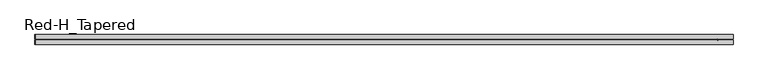
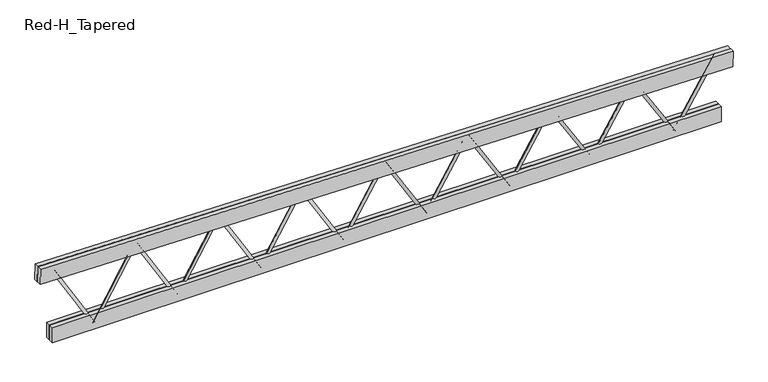
"""IFC4 building model written with IfcOpenShell, lengths in millimetres: beam geometry, Construction_Frames_RedBuilt_Openweb_Red-H_Tapered : Red-H_Tapered."""

import ifcopenshell
import ifcopenshell.guid

model = None  # the IFC model being written
_history = None  # IfcOwnerHistory: only IFC2X3 demands one
_inside = {}  # id of a spatial element -> (the spatial element, [elements in it])
_under = {}  # id of a project, library or spatial element -> (it, [spatial elements below it])
_declared = {}  # id of a project -> (the project, [libraries it declares])
_typed = {}  # id of a type object -> (the type object, [elements of that type])
_made_of = {}  # id of a material, layer set ... -> (it, [elements and type objects made of it])


def new_model(schema):
    """Start an empty IFC model of exactly this schema.

    Asked for "IFC4X3", IfcOpenShell would pick the latest addendum, in which some entities
    have other attributes; the version numbers below select the first issue.
    IFC2X3 requires an IfcOwnerHistory on every rooted entity: one is made here for all.
    """
    global model, _history
    if schema == "IFC4X3":
        model = ifcopenshell.file(schema_version=(4, 3, 0, 0))
    else:
        model = ifcopenshell.file(schema=schema)
    _inside.clear()
    _under.clear()
    _declared.clear()
    _typed.clear()
    _made_of.clear()
    _history = None
    if model.schema == "IFC2X3":
        org = make("IfcOrganization", Name="unknown")
        user = make(
            "IfcPersonAndOrganization",
            ThePerson=make("IfcPerson", FamilyName="unknown"),
            TheOrganization=org,
        )
        app = make(
            "IfcApplication",
            ApplicationDeveloper=org,
            Version="unknown",
            ApplicationFullName="unknown",
            ApplicationIdentifier="unknown",
        )
        _history = make(
            "IfcOwnerHistory",
            OwningUser=user,
            OwningApplication=app,
            ChangeAction="ADDED",
            CreationDate=0,
        )
    return model


def make(cls, **values):
    """One entity of the class cls with the attributes given. An attribute that is None is left unset."""
    return model.create_entity(
        cls, **{name: value for name, value in values.items() if value is not None}
    )


def rooted(cls, **values):
    """An entity with a GlobalId (a new one), such as an element, a storey or a relation."""
    return make(cls, GlobalId=ifcopenshell.guid.new(), OwnerHistory=_history, **values)


def si_unit(unit_type, name, prefix=None):
    """IfcSIUnit, for example si_unit("LENGTHUNIT", "METRE", prefix="MILLI")."""
    return make("IfcSIUnit", UnitType=unit_type, Prefix=prefix, Name=name)


def assignment(units):
    """IfcUnitAssignment: the units of a project."""
    return None if units is None else make("IfcUnitAssignment", Units=units)


def point(xyz):
    """IfcCartesianPoint."""
    return None if xyz is None else make("IfcCartesianPoint", Coordinates=xyz)


def direction(xyz):
    """IfcDirection."""
    return None if xyz is None else make("IfcDirection", DirectionRatios=xyz)


def frame(location, z_axis=None, x_axis=None):
    """IfcAxis2Placement3D, a coordinate frame: its origin and axes. An axis left out is left unset."""
    return make(
        "IfcAxis2Placement3D",
        Location=point(location),
        Axis=direction(z_axis),
        RefDirection=direction(x_axis),
    )


def frame_2d(location, x_axis=None):
    """IfcAxis2Placement2D, a coordinate frame in the plane: its origin and x axis."""
    return make(
        "IfcAxis2Placement2D", Location=point(location), RefDirection=direction(x_axis)
    )


def origin():
    """The frame at (0, 0, 0) with its axes left unset."""
    return frame((0.0, 0.0, 0.0))


def origin_2d():
    """The frame at (0, 0) in the plane with its x axis left unset."""
    return frame_2d((0.0, 0.0))


def place(relative_to, where):
    """IfcLocalPlacement: puts the frame where relative to a parent placement (None: the world)."""
    return make(
        "IfcLocalPlacement", PlacementRelTo=relative_to, RelativePlacement=where
    )


def context(
    kind, dimensions, precision=None, world=None, true_north=None, identifier=None
):
    """IfcGeometricRepresentationContext, for example the 3D "Model" context."""
    return make(
        "IfcGeometricRepresentationContext",
        ContextIdentifier=identifier,
        ContextType=kind,
        CoordinateSpaceDimension=dimensions,
        Precision=precision,
        WorldCoordinateSystem=world,
        TrueNorth=true_north,
    )


def project(units=None, contexts=None):
    """IfcProject with its units and contexts."""
    return rooted(
        "IfcProject",
        Name="project",
        RepresentationContexts=contexts,
        UnitsInContext=assignment(units),
    )


def spatial(cls, under=None, at=None, **own):
    """A site, building, storey or space (cls), placed at a placement, below another one or the project."""
    s = rooted(cls, ObjectPlacement=at, **own)
    if under is not None:
        _under.setdefault(under.id(), (under, []))[1].append(s)
    return s


def polyline(points):
    """IfcPolyline through the points."""
    return make("IfcPolyline", Points=[point(p) for p in points])


def circle_curve(where, radius):
    """IfcCircle in the frame where."""
    return make("IfcCircle", Position=where, Radius=radius)


def trimmed(basis, trim1, trim2, sense, master):
    """IfcTrimmedCurve: the piece of a basis curve between two trims."""
    return make(
        "IfcTrimmedCurve",
        BasisCurve=basis,
        Trim1=trim1,
        Trim2=trim2,
        SenseAgreement=sense,
        MasterRepresentation=master,
    )


def segment(curve, same_sense, transition):
    """IfcCompositeCurveSegment."""
    return make(
        "IfcCompositeCurveSegment",
        Transition=transition,
        SameSense=same_sense,
        ParentCurve=curve,
    )


def composite_curve(segments, self_intersect=None):
    """IfcCompositeCurve: segments joined end to end."""
    return make("IfcCompositeCurve", Segments=segments, SelfIntersect=self_intersect)


def outline(outer, holes=None, kind="AREA"):
    """IfcArbitraryClosedProfileDef: a profile drawn as a closed curve; with holes, ...WithVoids."""
    if holes is None:
        return make("IfcArbitraryClosedProfileDef", ProfileType=kind, OuterCurve=outer)
    return make(
        "IfcArbitraryProfileDefWithVoids",
        ProfileType=kind,
        OuterCurve=outer,
        InnerCurves=holes,
    )


def extrude(swept, where, along, depth):
    """IfcExtrudedAreaSolid: the profile swept, set in the frame where, extruded along a direction by depth."""
    return make(
        "IfcExtrudedAreaSolid",
        SweptArea=swept,
        Position=where,
        ExtrudedDirection=direction(along),
        Depth=depth,
    )


def shape(context_of_items, identifier, shape_type, items):
    """IfcShapeRepresentation: the items that make up one representation, for example the "Body"."""
    return make(
        "IfcShapeRepresentation",
        ContextOfItems=context_of_items,
        RepresentationIdentifier=identifier,
        RepresentationType=shape_type,
        Items=items,
    )


def source(mapping_origin, context_of_items, identifier, shape_type, items):
    """IfcRepresentationMap: a shape defined once, which mapped items show again and again."""
    return make(
        "IfcRepresentationMap",
        MappingOrigin=mapping_origin,
        MappedRepresentation=shape(context_of_items, identifier, shape_type, items),
    )


def transform(
    local_origin,
    x_axis=None,
    y_axis=None,
    z_axis=None,
    scale=None,
    scale2=None,
    scale3=None,
    uniform=True,
):
    """IfcCartesianTransformationOperator3D, or its non-uniform kind. x_axis, y_axis, z_axis: its Axis1, 2, 3."""
    if uniform:
        return make(
            "IfcCartesianTransformationOperator3D",
            Axis1=direction(x_axis),
            Axis2=direction(y_axis),
            LocalOrigin=point(local_origin),
            Scale=scale,
            Axis3=direction(z_axis),
        )
    return make(
        "IfcCartesianTransformationOperator3DnonUniform",
        Axis1=direction(x_axis),
        Axis2=direction(y_axis),
        LocalOrigin=point(local_origin),
        Scale=scale,
        Axis3=direction(z_axis),
        Scale2=scale2,
        Scale3=scale3,
    )


def mapped(mapping_source, mapping_target):
    """IfcMappedItem: shows the shape of a source again, moved by a transform."""
    return make(
        "IfcMappedItem", MappingSource=mapping_source, MappingTarget=mapping_target
    )


def made_of(thing, what):
    """Note that an element or type object is made of a material, layer set ...; save() writes the relation."""
    if what is not None:
        _made_of.setdefault(what.id(), (what, []))[1].append(thing)
    return thing


def element(
    cls,
    number,
    at=None,
    inside=None,
    cuts=None,
    type_object=None,
    material=None,
    context=None,
    identifier="Body",
    shape_type=None,
    held_by="IfcProductDefinitionShape",
    body=None,
    shapes=None,
    **own,
):
    """One element of the class cls, such as IfcWall. Its Tag is "e" and its number.

    at: its placement. inside: the storey or other place that contains it. cuts: it is an
    opening in that element (IfcRelVoidsElement). A single representation is given by context,
    identifier, shape_type and body (its items); several are given by shapes. held_by: the class
    of the entity that holds the representations. save() writes the other relations.
    """
    e = rooted(cls, Tag="e%d" % number, ObjectPlacement=at, **own)
    if body is not None:
        shapes = [shape(context, identifier, shape_type, body)]
    if shapes is not None:
        e.Representation = make(held_by, Representations=shapes)
    if inside is not None:
        _inside.setdefault(inside.id(), (inside, []))[1].append(e)
    if cuts is not None:
        rooted(
            "IfcRelVoidsElement", RelatingBuildingElement=cuts, RelatedOpeningElement=e
        )
    if type_object is not None:
        _typed.setdefault(type_object.id(), (type_object, []))[1].append(e)
    return made_of(e, material)


def aggregate(whole, parts):
    """IfcRelAggregates: a whole, such as a stair, and the parts it consists of."""
    return rooted("IfcRelAggregates", RelatingObject=whole, RelatedObjects=parts)


def save(model, path):
    """Write the relations noted so far, then the file.

    IfcRelAggregates (storeys below a building ...), IfcRelContainedInSpatialStructure (elements
    in a storey), IfcRelDefinesByType, IfcRelAssociatesMaterial and IfcRelDeclares: one each for
    every whole, place, type object, material and project.
    """
    for whole, parts in _under.values():
        aggregate(whole, parts)
    for where, things in _inside.values():
        rooted(
            "IfcRelContainedInSpatialStructure",
            RelatedElements=things,
            RelatingStructure=where,
        )
    for kind, things in _typed.values():
        rooted("IfcRelDefinesByType", RelatedObjects=things, RelatingType=kind)
    for what, things in _made_of.values():
        rooted("IfcRelAssociatesMaterial", RelatedObjects=things, RelatingMaterial=what)
    for by, libraries in _declared.values():
        rooted("IfcRelDeclares", RelatingContext=by, RelatedDefinitions=libraries)
    model.write(path)


def red_h_tapered_ce24421a(model_context):
    return source(origin(), model_context, "Body", "SweptSolid", [
        extrude(outline(composite_curve([segment(trimmed(circle_curve(origin_2d(), 12.7), [point((0.0, 12.7))], [point((0.0, -12.7))], False, "CARTESIAN"), True, "CONTINUOUS"), segment(trimmed(circle_curve(origin_2d(), 12.7), [point((0.0, -12.7))], [point((0.0, 12.7))], False, "CARTESIAN"), True, "CONTINUOUS")], self_intersect=False)), frame((2515.0014939, 0.0, -367.0101562), z_axis=(0.5238628746877267, 0.0, 0.8518026112450648), x_axis=(0.0, -1.0, 0.0)), (0.0, 0.0, 1.0), 685.8396444),
        extrude(outline(composite_curve([segment(trimmed(circle_curve(origin_2d(), 12.7), [point((0.0, -12.7000001))], [point((0.0, 12.7))], False, "CARTESIAN"), True, "CONTINUOUS"), segment(trimmed(circle_curve(origin_2d(), 12.7), [point((0.0, 12.7))], [point((0.0, -12.7000001))], False, "CARTESIAN"), True, "CONTINUOUS")], self_intersect=False)), frame((2515.0014939, 0.0, -367.0101562), z_axis=(-0.5212917882884671, 0.0, 0.8533785042189731), x_axis=(0.0, -1.0, 0.0)), (0.0, 0.0, 1.0), 689.2223046),
        extrude(outline(composite_curve([segment(trimmed(circle_curve(origin_2d(), 12.7), [point((0.0, 12.7))], [point((0.0, -12.7))], False, "CARTESIAN"), True, "CONTINUOUS"), segment(trimmed(circle_curve(origin_2d(), 12.7), [point((0.0, -12.7))], [point((0.0, 12.7))], False, "CARTESIAN"), True, "CONTINUOUS")], self_intersect=False)), frame((1796.4296385, 0.0, -367.0101562), z_axis=(0.5212917882884663, 0.0, 0.8533785042189738), x_axis=(0.0, -1.0, 0.0)), (0.0, 0.0, 1.0), 689.2223046),
        extrude(outline(composite_curve([segment(trimmed(circle_curve(origin_2d(), 12.7), [point((0.0, -12.7000001))], [point((0.0, 12.6999999))], False, "CARTESIAN"), True, "CONTINUOUS"), segment(trimmed(circle_curve(origin_2d(), 12.7), [point((0.0, 12.6999999))], [point((0.0, -12.7000001))], False, "CARTESIAN"), True, "CONTINUOUS")], self_intersect=False)), frame((1796.4296385, 0.0, -367.0101562), z_axis=(-0.5187411676162864, 0.0, 0.8549313428691757), x_axis=(0.0, -1.0, 0.0)), (0.0, 0.0, 1.0), 692.6111713),
        extrude(outline(composite_curve([segment(trimmed(circle_curve(origin_2d(), 12.7), [point((0.0, 12.7))], [point((0.0, -12.7))], False, "CARTESIAN"), True, "CONTINUOUS"), segment(trimmed(circle_curve(origin_2d(), 12.7), [point((0.0, -12.7))], [point((0.0, 12.7))], False, "CARTESIAN"), True, "CONTINUOUS")], self_intersect=False)), frame((1077.8577831, 0.0, -367.0101562), z_axis=(0.5187411676162853, 0.0, 0.8549313428691763), x_axis=(0.0, -1.0, 0.0)), (0.0, 0.0, 1.0), 692.6111713),
        extrude(outline(composite_curve([segment(trimmed(circle_curve(origin_2d(), 12.7), [point((0.0, -12.7))], [point((0.0, 12.7))], False, "CARTESIAN"), True, "CONTINUOUS"), segment(trimmed(circle_curve(origin_2d(), 12.7), [point((0.0, 12.7))], [point((0.0, -12.7))], False, "CARTESIAN"), True, "CONTINUOUS")], self_intersect=False)), frame((1077.8577831, 0.0, -367.0101562), z_axis=(-0.5162108492002061, 0.0, 0.8564615339686903), x_axis=(0.0, -1.0, 0.0)), (0.0, 0.0, 1.0), 696.0061538),
        extrude(outline(composite_curve([segment(trimmed(circle_curve(origin_2d(), 12.7), [point((0.0, 12.7))], [point((0.0, -12.7))], False, "CARTESIAN"), True, "CONTINUOUS"), segment(trimmed(circle_curve(origin_2d(), 12.7), [point((0.0, -12.7))], [point((0.0, 12.7))], False, "CARTESIAN"), True, "CONTINUOUS")], self_intersect=False)), frame((359.2859277, 0.0, -367.0101562), z_axis=(0.5162108492002068, 0.0, 0.85646153396869), x_axis=(0.0, -1.0, 0.0)), (0.0, 0.0, 1.0), 696.0061538),
        extrude(outline(composite_curve([segment(trimmed(circle_curve(origin_2d(), 12.7), [point((0.0, -12.7))], [point((0.0, 12.6999999))], False, "CARTESIAN"), True, "CONTINUOUS"), segment(trimmed(circle_curve(origin_2d(), 12.7), [point((0.0, 12.6999999))], [point((0.0, -12.7))], False, "CARTESIAN"), True, "CONTINUOUS")], self_intersect=False)), frame((359.2859277, 0.0, -367.0101562), z_axis=(-0.5137006691841376, 0.0, 0.8579694764266206), x_axis=(0.0, -1.0, 0.0)), (0.0, 0.0, 1.0), 699.4071631),
        extrude(outline(composite_curve([segment(trimmed(circle_curve(origin_2d(), 12.7), [point((0.0, -12.6999999))], [point((0.0, 12.7))], False, "CARTESIAN"), True, "CONTINUOUS"), segment(trimmed(circle_curve(origin_2d(), 12.7), [point((0.0, 12.7))], [point((0.0, -12.6999999))], False, "CARTESIAN"), True, "CONTINUOUS")], self_intersect=False)), frame((-359.2859277, 0.0, -367.0101562), z_axis=(0.5137006691841062, 0.0, 0.8579694764266393), x_axis=(0.0, -1.0, 0.0)), (0.0, 0.0, 1.0), 699.4071631),
        extrude(outline(composite_curve([segment(trimmed(circle_curve(origin_2d(), 12.7), [point((0.0, 12.6999999))], [point((0.0, -12.7))], False, "CARTESIAN"), True, "CONTINUOUS"), segment(trimmed(circle_curve(origin_2d(), 12.7), [point((0.0, -12.7))], [point((0.0, 12.6999999))], False, "CARTESIAN"), True, "CONTINUOUS")], self_intersect=False)), frame((-359.2859277, 0.0, -367.0101562), z_axis=(-0.5112104634271233, 0.0, 0.8594555614356254), x_axis=(0.0, -1.0, 0.0)), (0.0, 0.0, 1.0), 702.8141116),
        extrude(outline(composite_curve([segment(trimmed(circle_curve(origin_2d(), 12.7), [point((0.0, -12.6999999))], [point((0.0, 12.7000001))], False, "CARTESIAN"), True, "CONTINUOUS"), segment(trimmed(circle_curve(origin_2d(), 12.7), [point((0.0, 12.7000001))], [point((0.0, -12.6999999))], False, "CARTESIAN"), True, "CONTINUOUS")], self_intersect=False)), frame((-1077.8577831, 0.0, -367.0101562), z_axis=(0.5112104634271216, 0.0, 0.8594555614356263), x_axis=(0.0, -1.0, 0.0)), (0.0, 0.0, 1.0), 702.8141116),
        extrude(outline(composite_curve([segment(trimmed(circle_curve(origin_2d(), 12.7), [point((0.0, 12.7))], [point((0.0, -12.7))], False, "CARTESIAN"), True, "CONTINUOUS"), segment(trimmed(circle_curve(origin_2d(), 12.7), [point((0.0, -12.7))], [point((0.0, 12.7))], False, "CARTESIAN"), True, "CONTINUOUS")], self_intersect=False)), frame((-1077.8577831, 0.0, -367.0101562), z_axis=(-0.5087400675988173, 0.0, 0.8609201726173867), x_axis=(0.0, -1.0, 0.0)), (0.0, 0.0, 1.0), 706.2269135),
        extrude(outline(composite_curve([segment(trimmed(circle_curve(origin_2d(), 12.7), [point((0.0, -12.7))], [point((0.0, 12.7))], False, "CARTESIAN"), True, "CONTINUOUS"), segment(trimmed(circle_curve(origin_2d(), 12.7), [point((0.0, 12.7))], [point((0.0, -12.7))], False, "CARTESIAN"), True, "CONTINUOUS")], self_intersect=False)), frame((-1796.4296385, 0.0, -367.0101562), z_axis=(0.5087400675988304, 0.0, 0.8609201726173789), x_axis=(0.0, -1.0, 0.0)), (0.0, 0.0, 1.0), 706.2269135),
        extrude(outline(composite_curve([segment(trimmed(circle_curve(origin_2d(), 12.7), [point((0.0, 12.7))], [point((0.0, -12.7))], False, "CARTESIAN"), True, "CONTINUOUS"), segment(trimmed(circle_curve(origin_2d(), 12.7), [point((0.0, -12.7))], [point((0.0, 12.7))], False, "CARTESIAN"), True, "CONTINUOUS")], self_intersect=False)), frame((-1796.4296385, 0.0, -367.0101562), z_axis=(-0.5062893172698286, 0.0, 0.8623636861663707), x_axis=(0.0, -1.0, 0.0)), (0.0, 0.0, 1.0), 709.6454842),
        extrude(outline(composite_curve([segment(trimmed(circle_curve(origin_2d(), 12.7), [point((0.0, -12.7))], [point((0.0, 12.7000001))], False, "CARTESIAN"), True, "CONTINUOUS"), segment(trimmed(circle_curve(origin_2d(), 12.7), [point((0.0, 12.7000001))], [point((0.0, -12.7))], False, "CARTESIAN"), True, "CONTINUOUS")], self_intersect=False)), frame((-2515.0014939, 0.0, -367.0101562), z_axis=(0.506289317269817, 0.0, 0.8623636861663776), x_axis=(0.0, -1.0, 0.0)), (0.0, 0.0, 1.0), 709.6454842),
        extrude(outline(composite_curve([segment(trimmed(circle_curve(origin_2d(), 12.7), [point((0.0, 12.7))], [point((0.0, -12.7))], False, "CARTESIAN"), True, "CONTINUOUS"), segment(trimmed(circle_curve(origin_2d(), 12.7), [point((0.0, -12.7))], [point((0.0, 12.7))], False, "CARTESIAN"), True, "CONTINUOUS")], self_intersect=False)), frame((-2515.0014939, 0.0, -367.0101562), z_axis=(-0.5038580479976417, 0.0, 0.8637864709915329), x_axis=(0.0, -1.0, 0.0)), (0.0, 0.0, 1.0), 713.0697408),
        extrude(outline(polyline([(-2899.6874215, -41.275), (-2899.6874215, -3.175), (2899.6874215, -3.175), (2899.6874215, -41.275), (-2899.6874215, -41.275)])), frame((0.0, 0.0, -386.0601562), z_axis=(0.0, 0.0, 1.0), x_axis=(1.0, 0.0, 0.0)), (0.0, 0.0, 1.0), 139.7),
        extrude(outline(polyline([(-2899.6874215, 3.175), (-2899.6874215, 41.275), (2899.6874215, 41.275), (2899.6874215, 3.175), (-2899.6874215, 3.175)])), frame((0.0, 0.0, -386.0601562), z_axis=(0.0, 0.0, 1.0), x_axis=(1.0, 0.0, 0.0)), (0.0, 0.0, 1.0), 139.7),
        extrude(outline(polyline([(0.0, -38.1), (0.0, 0.0), (6003.4346259, 0.0), (6003.4346259, -38.1), (0.0, -38.1)])), frame((-3003.6516548, -3.175, 185.4598509), z_axis=(0.01692364560154548, 0.0, 0.9998567848544877), x_axis=(0.9998567848544877, 0.0, -0.01692364560154548)), (0.0, 0.0, 1.0), 139.7),
        extrude(outline(polyline([(0.0, -38.1), (0.0, 0.0), (6003.4346259, 0.0), (6003.4346259, -38.1), (0.0, -38.1)])), frame((-3003.6516548, 41.275, 185.4598509), z_axis=(0.01692364560154548, 0.0, 0.9998567848544877), x_axis=(0.9998567848544877, 0.0, -0.01692364560154548)), (0.0, 0.0, 1.0), 139.7),
    ])


if __name__ == "__main__":
    model = new_model("IFC4")
    model_context = context("Model", 3, world=origin())
    ifc_project = project(units=[si_unit("LENGTHUNIT", "METRE", prefix="MILLI")], contexts=[model_context])
    site = spatial("IfcSite", under=ifc_project)
    building = spatial("IfcBuilding", under=site)
    placement = place(None, origin())
    red_h_tapered_shape = red_h_tapered_ce24421a(model_context)
    element("IfcBeam", 1, ObjectType="Construction_Frames_RedBuilt_Openweb_Red-H_Tapered : Red-H_Tapered", at=placement, inside=building, context=model_context, shape_type="MappedRepresentation", body=[
        mapped(red_h_tapered_shape, transform((0.0, 0.0, 0.0), x_axis=(1.0, 0.0, 0.0), y_axis=(0.0, 1.0, 0.0), z_axis=(0.0, 0.0, 1.0))),
    ])
    save(model, "model.ifc")

# Revit data of these elements
# Type "Construction_Frames_RedBuilt_Openweb_Red-H_Tapered : Red-H_Tapered"
#   Youtube clip = ""
#   Weight Net (Kg) = "0"
#   Webs = "Up to 2\" diameter tubular steel"
#   Uniformat II Description = ""
#   Uniformat II Code = ""
#   Uniclass 2015 Name = "Softwood trusses"
#   Uniclass 2015 Code = "Pr_20_85_90_81"
#   Uniclass 2.0 Description = "Structural Framing Systems"
#   Uniclass 2.0 Code = "SS-15-10-75"
#   Uniclass 1.4 Description = "Trusses"
#   Uniclass 1.4 Code = "L3523"
#   UNSPSC Code = "30103606"
#   Technical description = "http://www.redbuilt.com/reference/literature-and-other-resources"
#   Region South America = "None"
#   Region Oceania = "None"
#   Region North America = "US"
#   Region Middle East = "None"
#   Region Europe = "None"
#   Region Asia = "None"
#   Region Antarctica = "None"
#   Region Africa = "None"
#   QR code = "http://bimobject.com/redbuilt/product/redbuilt-0003"
#   Product url = "http://www.redbuilt.com/products/default.aspx?id=2"
#   Product group = "Wood Trusses"
#   Product family = "Construction"
#   Product data url = "https://bimobject.com/redbuilt/product/redbuilt-0003"
#   Product certification = ""
#   Product SKU = "redbuilt-0003"
#   Product Page URL = "http://www.redbuilt.com/commercial-systems/red-m-red-h-open-web-trusses"
#   Product Guid = "2c5793f2-6ffb-4665-b825-cf90c048e711"
#   Product Documentation Link = "http://www.redbuilt.com/documents/OW_Guide_2017_07_LowRes_wLinks.pdf"
#   OmniClass Description = "Wood Trusses"
#   OmniClass Code = "23-13 35 19 13 17"
#   NBS Reference Description = ""
#   NBS Reference Code = ""
#   Material secondary = "Steel"
#   Material main = "CHARRED WOOD"
#   Masterformat 2014 Description = "Metal-Web Wood Joists"
#   Masterformat 2014 Code = "06 17 36"
#   Manufacturer name = "RedBuilt"
#   Manufacturer country = "United States"
#   Installation instructions = "http://www.redbuilt.com/documents/Installation_Sheets_Open-Web.pdf"
#   IFC Classification = ""
#   EAN code = ""
#   Design country = "United States"
#   Product Information = "http://redbuilt.com/products/default.aspx?id=2"
#   Model = "Red-H-Tapered"
#   Manufacturer URL = "http://redbuilt.com/"
#   Manufacturer = "RedBuilt™"
#   Description = "Open Web Truss"
#   Date of publishing = "8/17/2010"
#   Contact us = "http://redbuilt.com/contact/"
#   Chords = "Double 1½\" x 5½\" MSR lumber"
#   COBIe Type Category = ""
#   Brand url = "http://www.redbuilt.com"
#   BIMobject main category code = "construction"
#   BIMobject main category = "Construction"
#   BIMobject category code = "construction-frames-trusses"
#   BIMobject category = "Frames & Trusses"
#   Web Radius = 0' - 0 1/2"
#   Web Layout Offset Start [instance default] = 0' - 5"
#   Web Layout Offset End [instance default] = 0' - 5"
#   Web Diameter = 0' - 1"
#   TotalLength [instance default] = 20' - 0"
#   Span Minimum = 4' - 0"
#   Span Maximum = 70' - 0"
#   Span Limit [instance default] = 20' - 0"
#   Nominal width = 0' - 0"
#   Nominal height = 0' - 0"
#   Inner Depth Top [instance default] = 0' - 2.76372"
#   Depth Start [instance default] = 6' - 0"
#   Top Chord Length [instance default] = 20' - 1.19701"
#   TC Extension Start Aux [instance default] = 0' - 0"
#   TC Extension End Aux [instance default] = 0' - 0"
#   T-B Chord Length Difference L [instance default] = 0' - 4"
#   T-B Chord Length Difference [instance default] = 0' - 4"
#   Height 2 [instance default] = 6' - 0"
#   Depth Minimum at Wall = 2' - 0"
#   Depth Maximum at Wall = 6' - 0"
#   Depth Lower End [instance default] = 2' - 0"
#   Depth Higher End [instance default] = 6' - 0"
#   Depth End [instance default] = 2' - 0"
#   Depth 2 [instance default] = 2' - 0"
#   Chord Width = 0' - 3 1/4"
#   Chord Thickness = 0' - 1 1/2"
#   Chord Depth = 0' - 5 1/2"
#   Offset Start [instance default] = 0' - 0"
#   TC Extension Start [instance default] = 0' - 0"
#   End Panel = 0' - 5"
#   Offset End [instance default] = 0' - 0"
#   TC Extension End [instance default] = 0' - 0"
#   Length [instance default] = 20' - 0"
#   Angle [instance default] = 5.71059°
#   Span Limit Warning [instance default] = no
#   Edition number = 1
#   Top Bearing Start [instance default] = yes
#   Top Bearing End [instance default] = yes
#   Bottom Bearing Start [instance default] = no
#   Bottom Bearing End [instance default] = no
#   8 Panels [instance default] = yes
#   16 Panels [instance default] = no
#   12 Panels [instance default] = no
#   Web Material = RedBuilt-Steel, Galvanized
#   Clip Material = RedBuilt-Steel, Galvanized
#   Chords Material = WOOD-OAKFIRE
#   URL = ""
#   Assembly Code = ""
# Element 1 (IfcBeam, "Construction_Frames_RedBuilt_Openweb_Red-H_Tapered : Red-H_Tapered")
#   TotalLength = 19' - 8.32184"
#   Span Limit = 19' - 8.32184"
#   Inner Depth Top = 0' - 2.75039"
#   Depth Start = 5' - 0"
#   Top Chord Length = 19' - 8.35569"
#   Height 2 = 5' - 0"
#   Depth Higher End = 5' - 0"
#   Depth 2 = 0' - 4"
#   Angle = 0.9697°
#   Materials on its faces: "RedBuilt-Steel, Galvanized", "WOOD-OAKFIRE"
# Materials
#   "RedBuilt-Steel, Galvanized": class "Metal", colour RGB 164 172 176, transparency 0, Manufacturer = "RedBuilt. LLC", Comments = "Openweb Metal Web", URL = "http://www.redbuilt.com/", Description = "Galvanized steel", Cost = 0
#   "WOOD-OAKFIRE": class "Wood", colour RGB 198 202 183, transparency 0, Description = "Generic wood", Cost = 0
